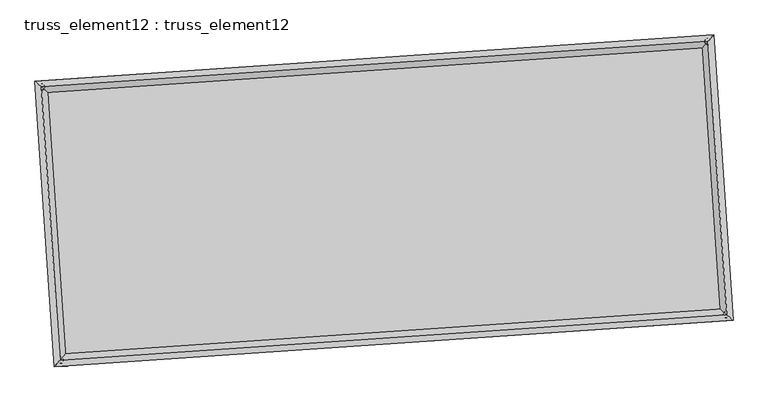
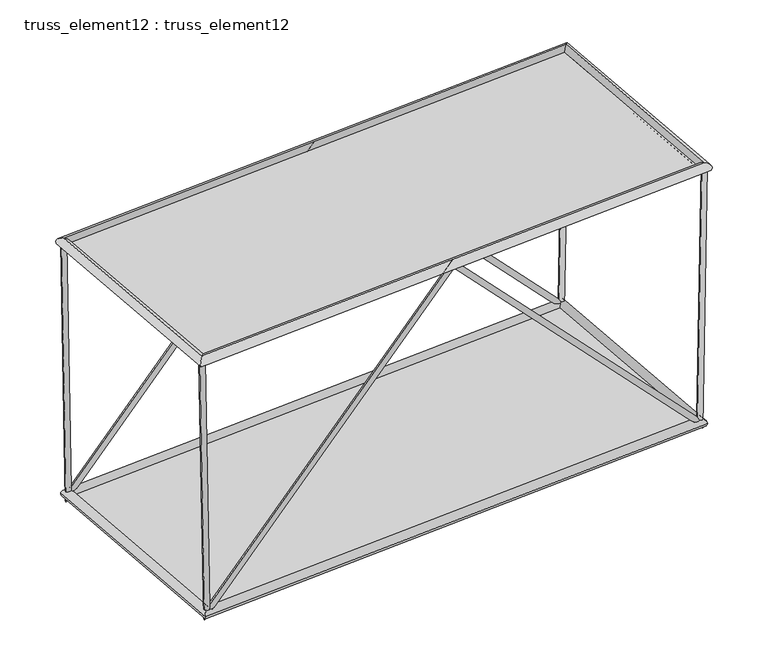
"""IFC4 building model written with IfcOpenShell, lengths in millimetres: plate geometry, truss_element12 : truss_element12."""

from ifc_helpers import new_model, si_unit, frame, origin, origin_with_axes, place, context, project, spatial, polyline, circle_curve, ellipse_curve, outline, extrude, source, transform, mapped, element, save
from ifc_brep_helpers import plane_surface, cylinder_surface, advanced_brep


def truss_element12_truss_element12_ae3a266e(model_context):
    return source(origin(), model_context, "Body", "SolidModel", [
        advanced_brep(
        [(-3756.1802311, 2270.0027691, 5000.0761995), (-3855.2669443, 2256.6426372, 4998.2513335), (-3667.1577697, 2276.0728724, 121.8875578), (-3761.8291131, 2263.0138077, -121.8875578), (1063.0031207, 2598.6045625, 5071.2944622), (1063.4620192, 2592.0320674, 4927.0589367), (5794.562368, 2921.2316012, 121.8973846), (5890.198609, 2921.1488873, -121.8973846), (5882.1969104, 2927.2070675, 5000.0878443), (5982.180545, 2927.4207859, 4998.2914205)],
        [
            (0, 1, circle_curve(frame((-3805.7235877, 2263.3227032, 4999.1637665), z_axis=(-0.01824602926340183, -0.0012441273758235993, 0.9998327532958659), x_axis=(-0.13360167870548645, 0.9910343786135793, -0.0012049286588313372)), 50.0)),
            (1, 0, circle_curve(frame((-3805.7235877, 2263.3227032, 4999.1637665), z_axis=(-0.01824602926340183, -0.0012441273758235993, 0.9998327532958659), x_axis=(-0.13360167870548645, 0.9910343786135793, -0.0012049286588313372)), 50.0)),
            (0, 2),
            (2, 3, ellipse_curve(frame((-3714.4934414, 2269.54334, 0.0), z_axis=(-0.9291499210086428, -0.06335520108406499, 0.3642341867332479), x_axis=(0.3633904003865977, 0.024778210026124285, 0.93130739136698)), 131.1628889, 50.0)),
            (3, 1),
            (3, 2, ellipse_curve(frame((-3714.4934414, 2269.54334, 0.0), z_axis=(-0.9291499210086428, -0.06335520108406499, 0.3642341867332479), x_axis=(0.3633904003865977, 0.024778210026124285, 0.93130739136698)), 131.1628889, 50.0)),
            (2, 4),
            (4, 5, ellipse_curve(frame((1063.23257, 2595.3183149, 4999.1766994), z_axis=(-0.9976833933192731, -0.06802823804080799, -7.432364115787789e-05), x_axis=(7.415146271864652e-05, 5.056106369626309e-06, -0.9999999972379982)), 72.2747993, 50.0)),
            (5, 3),
            (5, 4, ellipse_curve(frame((1063.23257, 2595.3183149, 4999.1766994), z_axis=(-0.9976833933192731, -0.06802823804080799, -7.432364115787789e-05), x_axis=(7.415146271864652e-05, 5.056106369626309e-06, -0.9999999972379982)), 72.2747993, 50.0)),
            (4, 6),
            (6, 7, ellipse_curve(frame((5842.3804885, 2921.1902443, 0.0), z_axis=(-0.9290710914132949, -0.06334982599361544, -0.36443614892966847), x_axis=(-0.36359189471660097, -0.02479194915854102, 0.9312283787306489)), 131.1845933, 50.0)),
            (7, 5),
            (7, 6, ellipse_curve(frame((5842.3804885, 2921.1902443, 0.0), z_axis=(-0.9290710914132949, -0.06334982599361544, -0.36443614892966847), x_axis=(-0.36359189471660097, -0.02479194915854102, 0.9312283787306489)), 131.1845933, 50.0)),
            (8, 9, circle_curve(frame((5932.1887277, 2927.3139267, 4999.1896324), z_axis=(0.01796164783284282, 0.0012247364871029384, 0.9998379264799202), x_axis=(-0.0021588384546528737, 0.99999696622927, -0.0011861487187809492)), 50.0)),
            (9, 8, circle_curve(frame((5932.1887277, 2927.3139267, 4999.1896324), z_axis=(0.01796164783284282, 0.0012247364871029384, 0.9998379264799202), x_axis=(-0.0021588384546528737, 0.99999696622927, -0.0011861487187809492)), 50.0)),
            (6, 8),
            (9, 7),
        ],
        [
            plane_surface(frame((-3805.7235877, 2313.3226645, 4999.2259832), z_axis=(-0.018246029263402925, -0.0012441273758274742, 0.999832753295866), x_axis=(0.9998335273514882, -2.270416412919475e-05, 0.01824601513760983))),
            cylinder_surface(frame((-3805.7235877, 2263.3227032, 4999.1637665), z_axis=(-0.018246029263401832, -0.0012441273758235995, 0.9998327532958661), x_axis=(-0.13360167870548645, 0.9910343786135793, -0.0012049286588313372)), 50.0),
            cylinder_surface(frame((-3714.4934414, 2269.54334, 0.0), z_axis=(-0.6901478836925812, -0.04705856069127947, -0.7221366840843337), x_axis=(-0.02041276416893784, 0.9987523004244808, -0.045575886780083084)), 50.0),
            cylinder_surface(frame((1063.23257, 2595.3183149, 4999.1766994), z_axis=(-0.6902549710503421, -0.04706586257113229, 0.7220338492901334), x_axis=(-0.11534133347445269, 0.992279482140813, -0.04558295859962826)), 50.0),
            plane_surface(frame((5932.1887277, 2877.3139642, 4999.2508791), z_axis=(0.017961647832841293, 0.001224736487099467, 0.9998379264799202), x_axis=(0.9998386765909434, -2.2001834880214226e-05, -0.017961634357437358))),
            cylinder_surface(frame((5842.3804885, 2921.1902443, 0.0), z_axis=(-0.01796164783284282, -0.0012247364871029384, -0.9998379264799202), x_axis=(-0.0021588384546528737, 0.99999696622927, -0.0011861487187809492)), 50.0),
        ],
        [
            (0, [[1, 2]]),
            (1, [[-1, 3, 4, 5]]),
            (1, [[-2, -5, 6, -3]]),
            (2, [[-4, 7, 8, 9]]),
            (2, [[-6, -9, 10, -7]]),
            (3, [[-8, 11, 12, 13]]),
            (3, [[-10, -13, 14, -11]]),
            (4, [[15, 16]]),
            (5, [[-12, 17, -16, 18]]),
            (5, [[-14, -18, -15, -17]]),
        ],
    ),
        advanced_brep(
        [(-3484.0672782, -1720.7308152, 5000.0761995), (-3583.1539914, -1734.0909471, 4998.2513335), (-3395.0448168, -1714.6607119, 121.8875578), (-3489.7161602, -1727.7197766, -121.8875578), (1335.1160737, -1392.1290218, 5071.2944622), (1335.5749721, -1398.7015169, 4927.0589367), (6066.6753209, -1069.5019831, 121.8973846), (6162.3115619, -1069.584697, -121.8973846), (6154.3098633, -1063.5265168, 5000.0878443), (6254.2934979, -1063.3127984, 4998.2914205)],
        [
            (0, 1, circle_curve(frame((-3533.6106348, -1727.4108811, 4999.1637665), z_axis=(-0.01824602926340309, -0.0012441273758237222, 0.9998327532958659), x_axis=(-0.1336016787054862, 0.9910343786135793, -0.0012049286588313795)), 50.0)),
            (1, 0, circle_curve(frame((-3533.6106348, -1727.4108811, 4999.1637665), z_axis=(-0.01824602926340309, -0.0012441273758237222, 0.9998327532958659), x_axis=(-0.1336016787054862, 0.9910343786135793, -0.0012049286588313795)), 50.0)),
            (0, 2),
            (2, 3, ellipse_curve(frame((-3442.3804885, -1721.1902443, 0.0), z_axis=(-0.9291499210086432, -0.06335520108406512, 0.364234186733247), x_axis=(0.3633904003865968, 0.024778210026124223, 0.9313073913669805)), 131.1628889, 50.0)),
            (3, 1),
            (3, 2, ellipse_curve(frame((-3442.3804885, -1721.1902443, 0.0), z_axis=(-0.9291499210086432, -0.06335520108406512, 0.364234186733247), x_axis=(0.3633904003865968, 0.024778210026124223, 0.9313073913669805)), 131.1628889, 50.0)),
            (2, 4),
            (4, 5, ellipse_curve(frame((1335.3455229, -1395.4152694, 4999.1766994), z_axis=(-0.9976833933192731, -0.06802823804080792, -7.432364116044547e-05), x_axis=(7.415146272126043e-05, 5.0561063696839735e-06, -0.999999997237998)), 72.2747993, 50.0)),
            (5, 3),
            (5, 4, ellipse_curve(frame((1335.3455229, -1395.4152694, 4999.1766994), z_axis=(-0.9976833933192731, -0.06802823804080792, -7.432364116044547e-05), x_axis=(7.415146272126043e-05, 5.0561063696839735e-06, -0.999999997237998)), 72.2747993, 50.0)),
            (4, 6),
            (6, 7, ellipse_curve(frame((6114.4934414, -1069.54334, 0.0), z_axis=(-0.9290710914132941, -0.06334982599361536, -0.3644361489296707), x_axis=(-0.363591894716603, -0.024791949158541025, 0.9312283787306479)), 131.1845933, 50.0)),
            (7, 5),
            (7, 6, ellipse_curve(frame((6114.4934414, -1069.54334, 0.0), z_axis=(-0.9290710914132941, -0.06334982599361536, -0.3644361489296707), x_axis=(-0.363591894716603, -0.024791949158541025, 0.9312283787306479)), 131.1845933, 50.0)),
            (8, 9, circle_curve(frame((6204.3016806, -1063.4196576, 4999.1896324), z_axis=(0.01796164783284177, 0.0012247364871029872, 0.9998379264799201), x_axis=(-0.0021588384546530333, 0.99999696622927, -0.0011861487187809978)), 50.0)),
            (9, 8, circle_curve(frame((6204.3016806, -1063.4196576, 4999.1896324), z_axis=(0.01796164783284177, 0.0012247364871029872, 0.9998379264799201), x_axis=(-0.0021588384546530333, 0.99999696622927, -0.0011861487187809978)), 50.0)),
            (6, 8),
            (9, 7),
        ],
        [
            plane_surface(frame((-3533.6106348, -1677.4109198, 4999.2259832), z_axis=(-0.018246029263402925, -0.0012441273758274944, 0.999832753295866), x_axis=(0.9998335273514882, -2.270416412919475e-05, 0.01824601513760983))),
            cylinder_surface(frame((-3533.6106348, -1727.4108811, 4999.1637665), z_axis=(-0.018246029263403095, -0.0012441273758237224, 0.9998327532958661), x_axis=(-0.1336016787054862, 0.9910343786135793, -0.0012049286588313795)), 50.0),
            cylinder_surface(frame((-3442.3804885, -1721.1902443, 0.0), z_axis=(-0.6901478836925803, -0.04705856069127945, -0.7221366840843344), x_axis=(-0.02041276416893806, 0.9987523004244808, -0.045575886780082814)), 50.0),
            cylinder_surface(frame((1335.3455229, -1395.4152694, 4999.1766994), z_axis=(-0.690254971050345, -0.04706586257113233, 0.7220338492901303), x_axis=(-0.11534133347445193, 0.992279482140813, -0.04558295859962813)), 50.0),
            plane_surface(frame((6204.3016806, -1113.4196201, 4999.2508791), z_axis=(0.017961647832841293, 0.001224736487099487, 0.9998379264799202), x_axis=(0.9998386765909434, -2.2001834880214226e-05, -0.017961634357437358))),
            cylinder_surface(frame((6114.4934414, -1069.54334, 0.0), z_axis=(-0.017961647832841772, -0.0012247364871029874, -0.9998379264799203), x_axis=(-0.0021588384546530333, 0.99999696622927, -0.0011861487187809978)), 50.0),
        ],
        [
            (0, [[1, 2]]),
            (1, [[-1, 3, 4, 5]]),
            (1, [[-2, -5, 6, -3]]),
            (2, [[-4, 7, 8, 9]]),
            (2, [[-6, -9, 10, -7]]),
            (3, [[-8, 11, 12, 13]]),
            (3, [[-10, -13, 14, -11]]),
            (4, [[15, 16]]),
            (5, [[-12, 17, -16, 18]]),
            (5, [[-14, -18, -15, -17]]),
        ],
    ),
        advanced_brep(
        [(-3533.6038857, -1727.4034009, 4909.1637668), (-3533.6173839, -1727.4183614, 5089.1637662), (-3805.7312897, 2263.3291981, 5089.1637662), (-3805.7158857, 2263.3162083, 4909.1637668), (5932.1950008, 2927.3213745, 5089.1896321), (5932.1824545, 2927.3064789, 4909.1896327), (6204.3089067, -1063.426185, 5089.1896321), (6204.2944545, -1063.4131303, 4909.1896327)],
        [
            (0, 1, ellipse_curve(frame((-3533.6106348, -1727.4108811, 4999.1637665), z_axis=(-0.7535719234029822, 0.6573654662782481, -1.8738715656892282e-06), x_axis=(-0.657365466275602, -0.7535719234052904, -1.8738715718147318e-06)), 127.2792206, 90.0)),
            (1, 2),
            (2, 3, ellipse_curve(frame((-3805.7235877, 2263.3227032, 4999.1637665), z_axis=(-0.657365466275602, -0.7535719234052904, -1.873871569304263e-06), x_axis=(0.7535719234029821, -0.6573654662782482, 1.8738715631787596e-06)), 127.2792206, 90.0)),
            (3, 0),
            (1, 0, ellipse_curve(frame((-3533.6106348, -1727.4108811, 4999.1637665), z_axis=(-0.7535719234029822, 0.6573654662782481, -1.8738715656892282e-06), x_axis=(-0.657365466275602, -0.7535719234052904, -1.8738715718147318e-06)), 127.2792206, 90.0)),
            (3, 2, ellipse_curve(frame((-3805.7235877, 2263.3227032, 4999.1637665), z_axis=(-0.657365466275602, -0.7535719234052904, -1.873871569304263e-06), x_axis=(0.7535719234029821, -0.6573654662782482, 1.8738715631787596e-06)), 127.2792206, 90.0)),
            (2, 4),
            (4, 5, ellipse_curve(frame((5932.1887277, 2927.3139267, 4999.1896324), z_axis=(-0.7535719234029844, 0.6573654662782455, -1.873871569304268e-06), x_axis=(-0.6573654662755994, -0.7535719234052927, -1.8738715631787545e-06)), 127.2792206, 90.0)),
            (5, 3),
            (5, 4, ellipse_curve(frame((5932.1887277, 2927.3139267, 4999.1896324), z_axis=(-0.7535719234029844, 0.6573654662782455, -1.873871569304268e-06), x_axis=(-0.6573654662755994, -0.7535719234052927, -1.8738715631787545e-06)), 127.2792206, 90.0)),
            (4, 6),
            (6, 7, ellipse_curve(frame((6204.3016806, -1063.4196576, 4999.1896324), z_axis=(0.6573654662755994, 0.7535719234052927, 1.8738715656892233e-06), x_axis=(-0.7535719234029844, 0.6573654662782457, -1.8738715718147367e-06)), 127.2792206, 90.0)),
            (7, 5),
            (7, 6, ellipse_curve(frame((6204.3016806, -1063.4196576, 4999.1896324), z_axis=(0.6573654662755994, 0.7535719234052927, 1.8738715656892233e-06), x_axis=(-0.7535719234029844, 0.6573654662782457, -1.8738715718147367e-06)), 127.2792206, 90.0)),
            (6, 1),
            (0, 7),
        ],
        [
            cylinder_surface(frame((-3533.6106348, -1727.4108811, 4999.1637665), z_axis=(0.06802823822870267, -0.9976833960748765, 0.0), x_axis=(-0.9976833928446474, -0.06802823800844562, -8.047023891255004e-05)), 90.0),
            cylinder_surface(frame((-3805.7235877, 2263.3227032, 4999.1637665), z_axis=(-0.9976833960713732, -0.0680282382284653, -2.6500545831240593e-06), x_axis=(-0.0680282378169653, 0.9976833930679299, -7.78201843331188e-05)), 90.0),
            cylinder_surface(frame((5932.1887277, 2927.3139267, 4999.1896324), z_axis=(-0.06802823822870929, 0.9976833960748762, 0.0), x_axis=(0.997683393256147, 0.06802823803651087, -7.517012975368756e-05)), 90.0),
            cylinder_surface(frame((6204.3016806, -1063.4196576, 4999.1896324), z_axis=(0.9976833960713731, 0.06802823822846524, 2.6500545866743975e-06), x_axis=(0.06802823822846522, -0.9976833930398712, -7.782018432800606e-05)), 90.0),
        ],
        [
            (0, [[1, 2, 3, 4]]),
            (0, [[5, -4, 6, -2]]),
            (1, [[-3, 7, 8, 9]]),
            (1, [[-6, -9, 10, -7]]),
            (2, [[-8, 11, 12, 13]]),
            (2, [[-10, -13, 14, -11]]),
            (3, [[-12, 15, -1, 16]]),
            (3, [[-14, -16, -5, -15]]),
        ],
    ),
        advanced_brep(
        [(-3358.7115243, -1625.2761972, 0.0), (-3526.0494527, -1817.1042913, 0.0), (-3810.4074885, 2353.2123043, 0.0), (-3618.5793943, 2185.8743758, 0.0), (5926.0494527, 3017.1042913, 0.0), (5758.7115243, 2825.2761972, 0.0), (6210.4074885, -1153.2123043, 0.0), (6018.5793943, -985.8743758, 0.0)],
        [
            (0, 1, ellipse_curve(frame((-3442.3804885, -1721.1902443, 0.0), z_axis=(-0.7535719234054582, 0.6573654662780805, 0.0), x_axis=(-0.6573654662780805, -0.7535719234054583, 0.0)), 127.2792206, 90.0)),
            (1, 2),
            (2, 3, ellipse_curve(frame((-3714.4934414, 2269.54334, 0.0), z_axis=(-0.6573654662780805, -0.7535719234054583, 0.0), x_axis=(0.7535719234054583, -0.6573654662780803, 0.0)), 127.2792206, 90.0)),
            (3, 0),
            (1, 0, ellipse_curve(frame((-3442.3804885, -1721.1902443, 0.0), z_axis=(-0.7535719234054582, 0.6573654662780805, 0.0), x_axis=(-0.6573654662780805, -0.7535719234054583, 0.0)), 127.2792206, 90.0)),
            (3, 2, ellipse_curve(frame((-3714.4934414, 2269.54334, 0.0), z_axis=(-0.6573654662780805, -0.7535719234054583, 0.0), x_axis=(0.7535719234054583, -0.6573654662780803, 0.0)), 127.2792206, 90.0)),
            (2, 4),
            (4, 5, ellipse_curve(frame((5842.3804885, 2921.1902443, 0.0), z_axis=(-0.7535719234054603, 0.657365466278078, 0.0), x_axis=(-0.6573654662780781, -0.7535719234054603, 0.0)), 127.2792206, 90.0)),
            (5, 3),
            (5, 4, ellipse_curve(frame((5842.3804885, 2921.1902443, 0.0), z_axis=(-0.7535719234054603, 0.657365466278078, 0.0), x_axis=(-0.6573654662780781, -0.7535719234054603, 0.0)), 127.2792206, 90.0)),
            (4, 6),
            (6, 7, ellipse_curve(frame((6114.4934414, -1069.54334, 0.0), z_axis=(0.6573654662780782, 0.7535719234054603, 0.0), x_axis=(-0.7535719234054604, 0.657365466278078, 0.0)), 127.2792206, 90.0)),
            (7, 5),
            (7, 6, ellipse_curve(frame((6114.4934414, -1069.54334, 0.0), z_axis=(0.6573654662780782, 0.7535719234054603, 0.0), x_axis=(-0.7535719234054604, 0.657365466278078, 0.0)), 127.2792206, 90.0)),
            (6, 1),
            (0, 7),
        ],
        [
            cylinder_surface(frame((-3442.3804885, -1721.1902443, 0.0), z_axis=(0.0680282382287011, -0.9976833960748767, 0.0), x_axis=(-0.9976833960748767, -0.0680282382287011, 0.0)), 90.0),
            cylinder_surface(frame((-3714.4934414, 2269.54334, 0.0), z_axis=(-0.9976833960748765, -0.06802823822870233, 0.0), x_axis=(-0.06802823822870233, 0.9976833960748765, 0.0)), 90.0),
            cylinder_surface(frame((5842.3804885, 2921.1902443, 0.0), z_axis=(-0.0680282382287075, 0.9976833960748761, 0.0), x_axis=(0.9976833960748761, 0.0680282382287075, 0.0)), 90.0),
            cylinder_surface(frame((6114.4934414, -1069.54334, 0.0), z_axis=(0.9976833960748767, 0.06802823822870217, 0.0), x_axis=(0.06802823822870217, -0.9976833960748767, 0.0)), 90.0),
        ],
        [
            (0, [[1, 2, 3, 4]]),
            (0, [[5, -4, 6, -2]]),
            (1, [[-3, 7, 8, 9]]),
            (1, [[-6, -9, 10, -7]]),
            (2, [[-8, 11, 12, 13]]),
            (2, [[-10, -13, 14, -11]]),
            (3, [[-12, 15, -1, 16]]),
            (3, [[-14, -16, -5, -15]]),
        ],
    ),
        extrude(outline(polyline([(-3442.3804885, -1721.1902443), (-3714.4934414, 2269.54334), (5842.3804885, 2921.1902443), (6114.4934414, -1069.54334), (-3442.3804885, -1721.1902443)])), origin_with_axes(), (0.0, 0.0, 1.0), 20.0),
        extrude(outline(polyline([(-2000.0, 4880.2617913), (2000.0, 4880.2617913), (2000.0, -4880.2617914), (-2000.0, -4880.2617914), (-2000.0, 4880.2617913)])), frame((1199.2890464, 599.9515228, 4999.1766994), z_axis=(-2.643915455980416e-06, -1.802785488212624e-07, 0.9999999999964887), x_axis=(-0.06802823822870048, 0.9976833960748767, 0.0)), (0.0, 0.0, 1.0), 20.0),
    ])


if __name__ == "__main__":
    model = new_model("IFC4")
    model_context = context("Model", 3, world=origin())
    ifc_project = project(units=[si_unit("LENGTHUNIT", "METRE", prefix="MILLI")], contexts=[model_context])
    site = spatial("IfcSite", under=ifc_project)
    building = spatial("IfcBuilding", under=site)
    placement = place(None, origin())
    truss_element12_truss_element12_shape = truss_element12_truss_element12_ae3a266e(model_context)
    element("IfcPlate", 1, ObjectType="truss_element12 : truss_element12", at=placement, inside=building, context=model_context, shape_type="MappedRepresentation", body=[
        mapped(truss_element12_truss_element12_shape, transform((0.0, 0.0, 0.0), x_axis=(1.0, 0.0, 0.0), y_axis=(0.0, 1.0, 0.0), z_axis=(0.0, 0.0, 1.0))),
    ])
    save(model, "model.ifc")

# Revit data of these elements
# Type "truss_element12 : truss_element12"
#   steellbar1 = 90 mm
#   steelbar2 = 50 mm
#   offset1 = 5000 mm
#   M = Default Roof
# Element 1 (IfcPlate, "truss_element12 : truss_element12")
#   Materials on its faces: "Default Roof"
# Materials
#   "Default Roof": class "Miscellaneous", colour RGB 0 127 0, transparency 0, Comments = "Rendering appearance not upgraded Rendering appearance not upgraded ", Cost = 0
